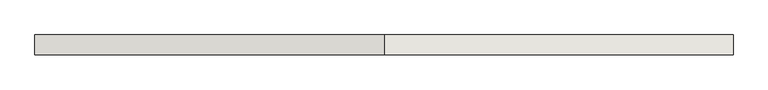
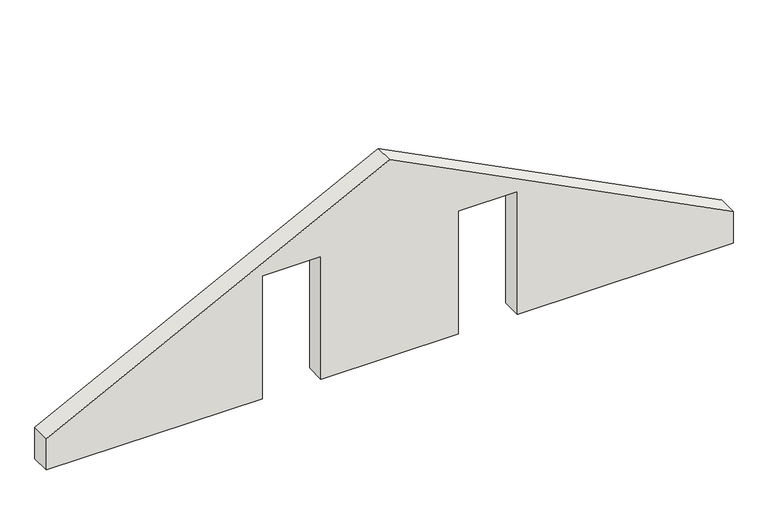
"""IFC4 building model written with IfcOpenShell, lengths in millimetres: wall geometry, 0_3d."""

from ifc_helpers import new_model, si_unit, frame, origin, place, context, project, spatial, polyline, outline, extrude, source, transform, mapped, element, save


def wall_f56b2bde(model_context):
    return source(origin(), model_context, "Body", "SweptSolid", [
        extrude(outline(polyline([(2500.0, 5295.0), (0.0, 5295.0), (0.0, 7945.0), (2500.0, 7945.0), (2500.0, 9080.0), (0.0, 9080.0), (0.0, 13240.0), (638.6196708, 13240.0), (4011.6781465, 6620.0), (638.6196708, 0.0), (0.0, 0.0), (0.0, 4160.0), (2500.0, 4160.0), (2500.0, 5295.0)])), frame((0.0, 0.0, 0.0), z_axis=(0.0, 1.0, 0.0), x_axis=(0.0, 0.0, 1.0)), (0.0, 0.0, 1.0), 380.0),
    ])


if __name__ == "__main__":
    model = new_model("IFC4")
    model_context = context("Model", 3, world=origin())
    ifc_project = project(units=[si_unit("LENGTHUNIT", "METRE", prefix="MILLI")], contexts=[model_context])
    site = spatial("IfcSite", under=ifc_project)
    building = spatial("IfcBuilding", under=site)
    placement = place(None, origin())
    wall_shape = wall_f56b2bde(model_context)
    element("IfcWall", 1, ObjectType="0_3d", at=placement, inside=building, context=model_context, shape_type="MappedRepresentation", body=[
        mapped(wall_shape, transform((0.0, 0.0, 0.0), x_axis=(1.0, 0.0, 0.0), y_axis=(0.0, 1.0, 0.0), z_axis=(0.0, 0.0, 1.0))),
    ])
    save(model, "model.ifc")

# Revit data of these elements
# Element 1 (IfcWall, "0_3d")
#   Materials on its faces: "holzschalung"
# Materials
#   "holzschalung": class "Unassigned", colour RGB 128 128 128, transparency 0
